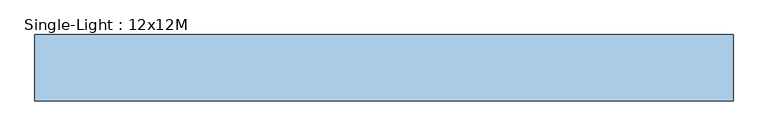
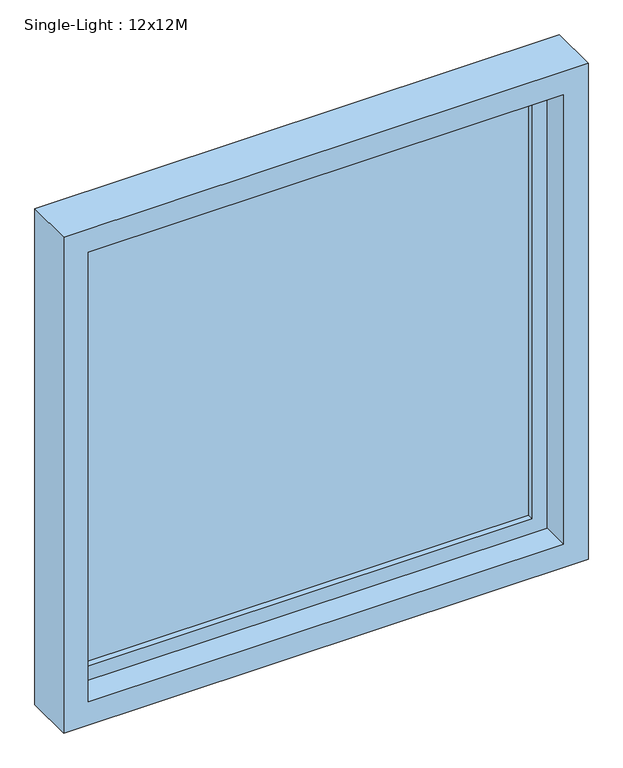
"""IFC4 building model written with IfcOpenShell, lengths in millimetres: window geometry, Single-Light : 12x12M."""

from ifc_helpers import new_model, si_unit, frame, origin, place, context, project, spatial, polyline, outline, extrude, faceted_brep, source, transform, mapped, element, save


def single_light_12x12m_8659da90(model_context):
    return source(origin(), model_context, "Body", "SolidModel", [
        extrude(outline(polyline([(1970.0, -564.0), (842.0, -564.0), (842.0, 564.0), (1970.0, 564.0), (1970.0, -564.0)]), holes=[polyline([(1920.0, 514.0), (892.0, 514.0), (892.0, -514.0), (1920.0, -514.0), (1920.0, 514.0)])]), frame((0.0, 134.0, 0.0), z_axis=(0.0, 1.0, 0.0), x_axis=(0.0, 0.0, 1.0)), (0.0, 0.0, 1.0), 50.0),
        faceted_brep([(-606.0, 69.0, 800.0), (-606.0, 184.0, 800.0), (606.0, 184.0, 800.0), (606.0, 69.0, 800.0), (606.0, 184.0, 2012.0), (606.0, 69.0, 2012.0), (-606.0, 184.0, 2012.0), (564.0, 184.0, 1970.0), (-564.0, 184.0, 1970.0), (-564.0, 184.0, 842.0), (564.0, 184.0, 842.0), (-606.0, 69.0, 2012.0), (549.0, 69.0, 857.0), (-549.0, 69.0, 857.0), (-549.0, 69.0, 1955.0), (549.0, 69.0, 1955.0), (-549.0, 134.0, 857.0), (549.0, 134.0, 857.0), (549.0, 134.0, 1955.0), (564.0, 134.0, 842.0), (-564.0, 134.0, 842.0), (-564.0, 134.0, 1970.0), (564.0, 134.0, 1970.0), (-549.0, 134.0, 1955.0)], [[[0, 1, 2, 3]], [[3, 2, 4, 5]], [[2, 1, 6, 4], [7, 8, 9, 10]], [[5, 11, 0, 3], [12, 13, 14, 15]], [[16, 13, 12, 17]], [[17, 12, 15, 18]], [[19, 20, 21, 22], [18, 23, 16, 17]], [[9, 20, 19, 10]], [[10, 19, 22, 7]], [[11, 6, 1, 0]], [[23, 14, 13, 16]], [[8, 21, 20, 9]], [[5, 4, 6, 11]], [[18, 15, 14, 23]], [[7, 22, 21, 8]]]),
        extrude(outline(polyline([(-514.0, 170.0), (514.0, 170.0), (514.0, 148.0), (-514.0, 148.0), (-514.0, 170.0)])), frame((0.0, 0.0, 892.0), z_axis=(0.0, 0.0, 1.0), x_axis=(1.0, 0.0, 0.0)), (0.0, 0.0, 1.0), 1028.0),
    ])


if __name__ == "__main__":
    model = new_model("IFC4")
    model_context = context("Model", 3, world=origin())
    ifc_project = project(units=[si_unit("LENGTHUNIT", "METRE", prefix="MILLI")], contexts=[model_context])
    site = spatial("IfcSite", under=ifc_project)
    building = spatial("IfcBuilding", under=site)
    placement = place(None, origin())
    single_light_12x12m_shape = single_light_12x12m_8659da90(model_context)
    element("IfcWindow", 1, ObjectType="Single-Light : 12x12M", at=placement, inside=building, context=model_context, shape_type="MappedRepresentation", body=[
        mapped(single_light_12x12m_shape, transform((0.0, 0.0, 0.0), x_axis=(1.0, 0.0, 0.0), y_axis=(0.0, 1.0, 0.0), z_axis=(0.0, 0.0, 1.0))),
    ])
    save(model, "model.ifc")

# Revit data of these elements
# Type "Single-Light : 12x12M"
#   Type Mark = "39"
#   Creator Organization [instance default] = "© Danish Educational Content"
#   Creator Name [instance default] = "© Erik Falck Jørgensen"
#   Creator Build [instance default] = "2017.0801.0"
#   Analytic Construction = "<None>"
#   length#5 = -36 mm
#   length#4 = -14 mm
#   length#3 = 120 mm
#   length#2 = 57 mm
#   length#1 = 0 mm
#   Seal Width = 12 mm
#   Rough Width = 1212 mm
#   Rough Height = 1212 mm
#   Rebate Depth = 50 mm
#   Rabbet Width = 15 mm
#   Rabbet Depth = 50 mm
#   Height = 1188 mm
#   Glass Thickness = 22 mm
#   Frame Width = 50 mm
#   Frame Depth = 50 mm
#   Exterior Direction [instance default] = 0.00°
#   Case Depth = 115 mm
#   Case Width = 45 mm
#   Default Sill Height = 800 mm
#   Width = 1188 mm
#   Sealing = no
#   Hinging = yes
#   Wall Closure = 1
#   Above Cutplane [instance default] = no
#   Wall Surface = none
#   Sill Plate = none
#   Glass = none
#   Frame/Mullion = none
#   Embrasure = none
#   Case/Transom = none
# Element 1 (IfcWindow, "Single-Light : 12x12M")
#   Materials on its faces: "Default Frame/Mullion (Interior/Exterior)", "Glass"
# Materials
#   "Default Frame/Mullion (Interior/Exterior)": class "Generic", colour RGB 205 205 205, transparency 0, Description = "Udefineret karm/ramme materiale", Cost = 0
#   "Glass": class "Glass", colour RGB 180 200 255, transparency 0.75, Description = "Generisk glas", Cost = 0
